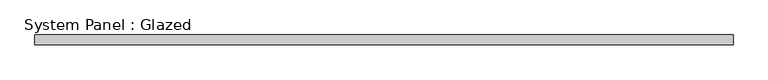
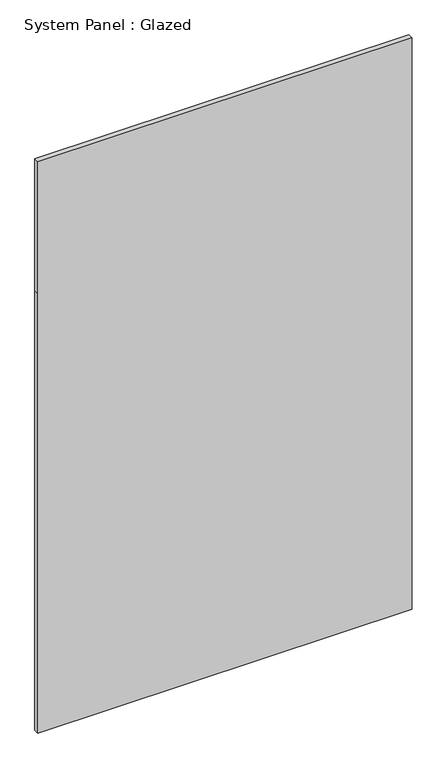
"""IFC4 building model written with IfcOpenShell, lengths in millimetres: plate geometry, System Panel : Glazed."""

from ifc_helpers import new_model, si_unit, frame, origin, place, context, project, spatial, polyline, outline, extrude, source, transform, mapped, element, save


def system_panel_glazed_67f2b0f9(model_context):
    return source(origin(), model_context, "Body", "SweptSolid", [
        extrude(outline(polyline([(0.0, -906.9444446), (0.0, 906.9444446), (2250.0, 906.9444446), (2925.0, 906.9444446), (2925.0, -906.9444446), (2250.0, -906.9444446), (0.0, -906.9444446)])), frame((0.0, 24.5, 0.0), z_axis=(0.0, 1.0, 0.0), x_axis=(0.0, 0.0, 1.0)), (0.0, 0.0, 1.0), 25.0),
    ])


if __name__ == "__main__":
    model = new_model("IFC4")
    model_context = context("Model", 3, world=origin())
    ifc_project = project(units=[si_unit("LENGTHUNIT", "METRE", prefix="MILLI")], contexts=[model_context])
    site = spatial("IfcSite", under=ifc_project)
    building = spatial("IfcBuilding", under=site)
    placement = place(None, origin())
    system_panel_glazed_shape = system_panel_glazed_67f2b0f9(model_context)
    element("IfcPlate", 1, ObjectType="System Panel : Glazed", at=placement, inside=building, context=model_context, shape_type="MappedRepresentation", body=[
        mapped(system_panel_glazed_shape, transform((0.0, 0.0, 0.0), x_axis=(1.0, 0.0, 0.0), y_axis=(0.0, 1.0, 0.0), z_axis=(0.0, 0.0, 1.0))),
    ])
    save(model, "model.ifc")

# Revit data of these elements
# Element 1 (IfcPlate, "System Panel : Glazed")
#   Materials on its faces: "Glass"
# Materials
#   "Glass": class "Glass", colour RGB 0 128 192, transparency 0.9
